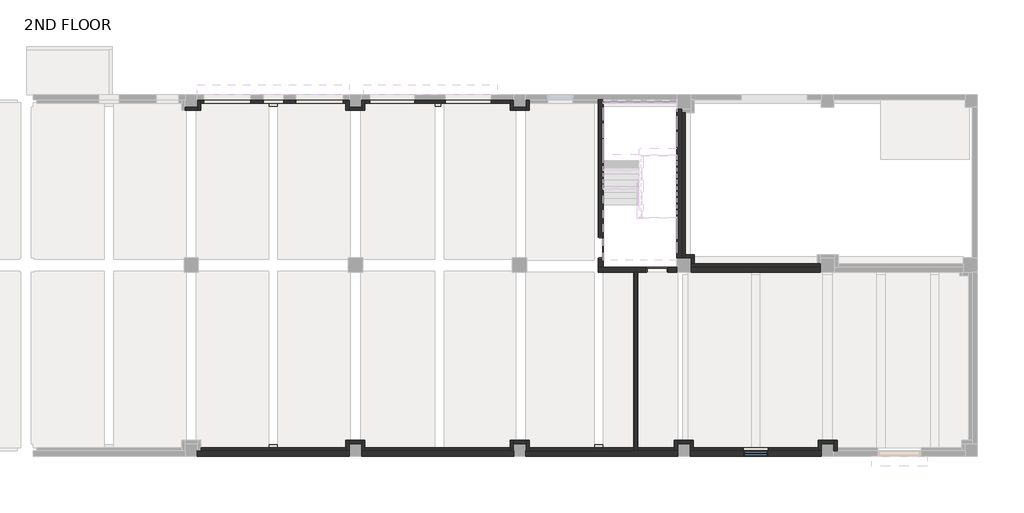
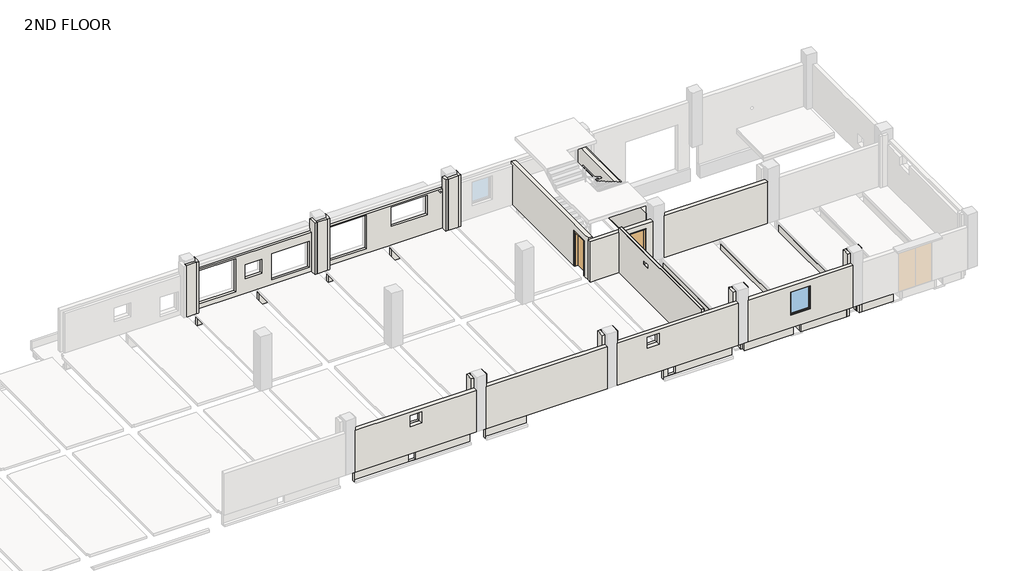
# One storey, part 2 of 7: 60 walls, 2 doors, 1 window.
"""IFC4 building model written with IfcOpenShell, lengths in millimetres."""

import ifcopenshell
import ifcopenshell.guid

model = None  # the IFC model being written
_history = None  # IfcOwnerHistory: only IFC2X3 demands one
_inside = {}  # id of a spatial element -> (the spatial element, [elements in it])
_under = {}  # id of a project, library or spatial element -> (it, [spatial elements below it])
_declared = {}  # id of a project -> (the project, [libraries it declares])
_typed = {}  # id of a type object -> (the type object, [elements of that type])
_made_of = {}  # id of a material, layer set ... -> (it, [elements and type objects made of it])


def new_model(schema):
    """Start an empty IFC model of exactly this schema.

    Asked for "IFC4X3", IfcOpenShell would pick the latest addendum, in which some entities
    have other attributes; the version numbers below select the first issue.
    IFC2X3 requires an IfcOwnerHistory on every rooted entity: one is made here for all.
    """
    global model, _history
    if schema == "IFC4X3":
        model = ifcopenshell.file(schema_version=(4, 3, 0, 0))
    else:
        model = ifcopenshell.file(schema=schema)
    _inside.clear()
    _under.clear()
    _declared.clear()
    _typed.clear()
    _made_of.clear()
    _history = None
    if model.schema == "IFC2X3":
        org = make("IfcOrganization", Name="unknown")
        user = make(
            "IfcPersonAndOrganization",
            ThePerson=make("IfcPerson", FamilyName="unknown"),
            TheOrganization=org,
        )
        app = make(
            "IfcApplication",
            ApplicationDeveloper=org,
            Version="unknown",
            ApplicationFullName="unknown",
            ApplicationIdentifier="unknown",
        )
        _history = make(
            "IfcOwnerHistory",
            OwningUser=user,
            OwningApplication=app,
            ChangeAction="ADDED",
            CreationDate=0,
        )
    return model


def make(cls, **values):
    """One entity of the class cls with the attributes given. An attribute that is None is left unset."""
    return model.create_entity(
        cls, **{name: value for name, value in values.items() if value is not None}
    )


def rooted(cls, **values):
    """An entity with a GlobalId (a new one), such as an element, a storey or a relation."""
    return make(cls, GlobalId=ifcopenshell.guid.new(), OwnerHistory=_history, **values)


def si_unit(unit_type, name, prefix=None):
    """IfcSIUnit, for example si_unit("LENGTHUNIT", "METRE", prefix="MILLI")."""
    return make("IfcSIUnit", UnitType=unit_type, Prefix=prefix, Name=name)


def assignment(units):
    """IfcUnitAssignment: the units of a project."""
    return None if units is None else make("IfcUnitAssignment", Units=units)


def point(xyz):
    """IfcCartesianPoint."""
    return None if xyz is None else make("IfcCartesianPoint", Coordinates=xyz)


def direction(xyz):
    """IfcDirection."""
    return None if xyz is None else make("IfcDirection", DirectionRatios=xyz)


def frame(location, z_axis=None, x_axis=None):
    """IfcAxis2Placement3D, a coordinate frame: its origin and axes. An axis left out is left unset."""
    return make(
        "IfcAxis2Placement3D",
        Location=point(location),
        Axis=direction(z_axis),
        RefDirection=direction(x_axis),
    )


def frame_2d(location, x_axis=None):
    """IfcAxis2Placement2D, a coordinate frame in the plane: its origin and x axis."""
    return make(
        "IfcAxis2Placement2D", Location=point(location), RefDirection=direction(x_axis)
    )


def origin():
    """The frame at (0, 0, 0) with its axes left unset."""
    return frame((0.0, 0.0, 0.0))


def origin_with_axes():
    """The frame at (0, 0, 0) with the z axis (0, 0, 1) and the x axis (1, 0, 0) written out."""
    return frame((0.0, 0.0, 0.0), z_axis=(0.0, 0.0, 1.0), x_axis=(1.0, 0.0, 0.0))


def place(relative_to, where):
    """IfcLocalPlacement: puts the frame where relative to a parent placement (None: the world)."""
    return make(
        "IfcLocalPlacement", PlacementRelTo=relative_to, RelativePlacement=where
    )


def context(
    kind, dimensions, precision=None, world=None, true_north=None, identifier=None
):
    """IfcGeometricRepresentationContext, for example the 3D "Model" context."""
    return make(
        "IfcGeometricRepresentationContext",
        ContextIdentifier=identifier,
        ContextType=kind,
        CoordinateSpaceDimension=dimensions,
        Precision=precision,
        WorldCoordinateSystem=world,
        TrueNorth=true_north,
    )


def project(units=None, contexts=None):
    """IfcProject with its units and contexts."""
    return rooted(
        "IfcProject",
        Name="project",
        RepresentationContexts=contexts,
        UnitsInContext=assignment(units),
    )


def spatial(cls, under=None, at=None, **own):
    """A site, building, storey or space (cls), placed at a placement, below another one or the project."""
    s = rooted(cls, ObjectPlacement=at, **own)
    if under is not None:
        _under.setdefault(under.id(), (under, []))[1].append(s)
    return s


def polyline(points):
    """IfcPolyline through the points."""
    return make("IfcPolyline", Points=[point(p) for p in points])


def circle_curve(where, radius):
    """IfcCircle in the frame where."""
    return make("IfcCircle", Position=where, Radius=radius)


def trimmed(basis, trim1, trim2, sense, master):
    """IfcTrimmedCurve: the piece of a basis curve between two trims."""
    return make(
        "IfcTrimmedCurve",
        BasisCurve=basis,
        Trim1=trim1,
        Trim2=trim2,
        SenseAgreement=sense,
        MasterRepresentation=master,
    )


def segment(curve, same_sense, transition):
    """IfcCompositeCurveSegment."""
    return make(
        "IfcCompositeCurveSegment",
        Transition=transition,
        SameSense=same_sense,
        ParentCurve=curve,
    )


def composite_curve(segments, self_intersect=None):
    """IfcCompositeCurve: segments joined end to end."""
    return make("IfcCompositeCurve", Segments=segments, SelfIntersect=self_intersect)


def outline(outer, holes=None, kind="AREA"):
    """IfcArbitraryClosedProfileDef: a profile drawn as a closed curve; with holes, ...WithVoids."""
    if holes is None:
        return make("IfcArbitraryClosedProfileDef", ProfileType=kind, OuterCurve=outer)
    return make(
        "IfcArbitraryProfileDefWithVoids",
        ProfileType=kind,
        OuterCurve=outer,
        InnerCurves=holes,
    )


def extrude(swept, where, along, depth):
    """IfcExtrudedAreaSolid: the profile swept, set in the frame where, extruded along a direction by depth."""
    return make(
        "IfcExtrudedAreaSolid",
        SweptArea=swept,
        Position=where,
        ExtrudedDirection=direction(along),
        Depth=depth,
    )


def faces_of(points, faces, orient=None, outer=None):
    """IfcFace entities. A face is a list of loops; a loop is a list of indices into points, from 0.

    orient and outer hold one flag for each loop. By default every Orientation is true, the
    first loop of a face is its IfcFaceOuterBound and the others are IfcFaceBound.
    """
    made = []
    for i, loops in enumerate(faces):
        bounds = []
        for j, loop in enumerate(loops):
            is_outer = j == 0 if outer is None else outer[i][j]
            bounds.append(
                make(
                    "IfcFaceOuterBound" if is_outer else "IfcFaceBound",
                    Bound=make("IfcPolyLoop", Polygon=[points[k] for k in loop]),
                    Orientation=True if orient is None else orient[i][j],
                )
            )
        made.append(make("IfcFace", Bounds=bounds))
    return made


def faceted_brep(points, faces, orient=None, outer=None, voids=None):
    """IfcFacetedBrep: a solid bounded by flat faces; with voids (closed shells), ...WithVoids."""
    shared = [point(p) for p in points]
    hull = make("IfcClosedShell", CfsFaces=faces_of(shared, faces, orient, outer))
    if voids is None:
        return make("IfcFacetedBrep", Outer=hull)
    return make(
        "IfcFacetedBrepWithVoids",
        Outer=hull,
        Voids=[
            make(cls, CfsFaces=faces_of(shared, fs, o, b)) for cls, fs, o, b in voids
        ],
    )


def shape(context_of_items, identifier, shape_type, items):
    """IfcShapeRepresentation: the items that make up one representation, for example the "Body"."""
    return make(
        "IfcShapeRepresentation",
        ContextOfItems=context_of_items,
        RepresentationIdentifier=identifier,
        RepresentationType=shape_type,
        Items=items,
    )


def source(mapping_origin, context_of_items, identifier, shape_type, items):
    """IfcRepresentationMap: a shape defined once, which mapped items show again and again."""
    return make(
        "IfcRepresentationMap",
        MappingOrigin=mapping_origin,
        MappedRepresentation=shape(context_of_items, identifier, shape_type, items),
    )


def transform(
    local_origin,
    x_axis=None,
    y_axis=None,
    z_axis=None,
    scale=None,
    scale2=None,
    scale3=None,
    uniform=True,
):
    """IfcCartesianTransformationOperator3D, or its non-uniform kind. x_axis, y_axis, z_axis: its Axis1, 2, 3."""
    if uniform:
        return make(
            "IfcCartesianTransformationOperator3D",
            Axis1=direction(x_axis),
            Axis2=direction(y_axis),
            LocalOrigin=point(local_origin),
            Scale=scale,
            Axis3=direction(z_axis),
        )
    return make(
        "IfcCartesianTransformationOperator3DnonUniform",
        Axis1=direction(x_axis),
        Axis2=direction(y_axis),
        LocalOrigin=point(local_origin),
        Scale=scale,
        Axis3=direction(z_axis),
        Scale2=scale2,
        Scale3=scale3,
    )


def mapped(mapping_source, mapping_target):
    """IfcMappedItem: shows the shape of a source again, moved by a transform."""
    return make(
        "IfcMappedItem", MappingSource=mapping_source, MappingTarget=mapping_target
    )


def made_of(thing, what):
    """Note that an element or type object is made of a material, layer set ...; save() writes the relation."""
    if what is not None:
        _made_of.setdefault(what.id(), (what, []))[1].append(thing)
    return thing


def element(
    cls,
    number,
    at=None,
    inside=None,
    cuts=None,
    type_object=None,
    material=None,
    context=None,
    identifier="Body",
    shape_type=None,
    held_by="IfcProductDefinitionShape",
    body=None,
    shapes=None,
    **own,
):
    """One element of the class cls, such as IfcWall. Its Tag is "e" and its number.

    at: its placement. inside: the storey or other place that contains it. cuts: it is an
    opening in that element (IfcRelVoidsElement). A single representation is given by context,
    identifier, shape_type and body (its items); several are given by shapes. held_by: the class
    of the entity that holds the representations. save() writes the other relations.
    """
    e = rooted(cls, Tag="e%d" % number, ObjectPlacement=at, **own)
    if body is not None:
        shapes = [shape(context, identifier, shape_type, body)]
    if shapes is not None:
        e.Representation = make(held_by, Representations=shapes)
    if inside is not None:
        _inside.setdefault(inside.id(), (inside, []))[1].append(e)
    if cuts is not None:
        rooted(
            "IfcRelVoidsElement", RelatingBuildingElement=cuts, RelatedOpeningElement=e
        )
    if type_object is not None:
        _typed.setdefault(type_object.id(), (type_object, []))[1].append(e)
    return made_of(e, material)


def aggregate(whole, parts):
    """IfcRelAggregates: a whole, such as a stair, and the parts it consists of."""
    return rooted("IfcRelAggregates", RelatingObject=whole, RelatedObjects=parts)


def save(model, path):
    """Write the relations noted so far, then the file.

    IfcRelAggregates (storeys below a building ...), IfcRelContainedInSpatialStructure (elements
    in a storey), IfcRelDefinesByType, IfcRelAssociatesMaterial and IfcRelDeclares: one each for
    every whole, place, type object, material and project.
    """
    for whole, parts in _under.values():
        aggregate(whole, parts)
    for where, things in _inside.values():
        rooted(
            "IfcRelContainedInSpatialStructure",
            RelatedElements=things,
            RelatingStructure=where,
        )
    for kind, things in _typed.values():
        rooted("IfcRelDefinesByType", RelatedObjects=things, RelatingType=kind)
    for what, things in _made_of.values():
        rooted("IfcRelAssociatesMaterial", RelatedObjects=things, RelatingMaterial=what)
    for by, libraries in _declared.values():
        rooted("IfcRelDeclares", RelatingContext=by, RelatedDefinitions=libraries)
    model.write(path)


def single_door_steel_8b0dfbf3(model_context):
    return source(origin(), model_context, "Body", "SolidModel", [
        extrude(outline(polyline([(505.0, -125.0), (-505.0, -125.0), (-505.0, -85.0), (505.0, -85.0), (505.0, -125.0)])), origin_with_axes(), (0.0, 0.0, 1.0), 2235.0),
        faceted_brep([(505.0, -125.0, 0.0), (505.0, -85.0, 0.0), (485.0, -85.0, 0.0), (485.0, 85.0, 0.0), (505.0, 85.0, 0.0), (505.0, 125.0, 0.0), (535.0, 125.0, 0.0), (535.0, -125.0, 0.0), (-505.0, -125.0, 0.0), (-535.0, -125.0, 0.0), (-535.0, 125.0, 0.0), (-505.0, 125.0, 0.0), (-505.0, 85.0, 0.0), (-485.0, 85.0, 0.0), (-485.0, -85.0, 0.0), (-505.0, -85.0, 0.0), (535.0, -125.0, 2265.0), (-535.0, -125.0, 2265.0), (-505.0, -125.0, 2235.0), (505.0, -125.0, 2235.0), (535.0, 125.0, 2265.0), (505.0, 125.0, 2235.0), (-505.0, 125.0, 2235.0), (-535.0, 125.0, 2265.0), (505.0, 85.0, 2235.0), (485.0, 85.0, 2215.0), (-485.0, 85.0, 2215.0), (-505.0, 85.0, 2235.0), (485.0, -85.0, 2215.0), (505.0, -85.0, 2235.0), (-505.0, -85.0, 2235.0), (-485.0, -85.0, 2215.0)], [[[0, 1, 2, 3, 4, 5, 6, 7]], [[8, 9, 10, 11, 12, 13, 14, 15]], [[7, 16, 17, 9, 8, 18, 19, 0]], [[6, 20, 16, 7]], [[5, 21, 22, 11, 10, 23, 20, 6]], [[4, 24, 21, 5]], [[3, 25, 26, 13, 12, 27, 24, 4]], [[2, 28, 25, 3]], [[1, 29, 30, 15, 14, 31, 28, 2]], [[0, 19, 29, 1]], [[18, 8, 15, 30]], [[23, 10, 9, 17]], [[27, 12, 11, 22]], [[31, 14, 13, 26]], [[20, 23, 17, 16]], [[24, 27, 22, 21]], [[28, 31, 26, 25]], [[19, 18, 30, 29]]]),
    ])


def fixed_window_c6e05aa5(model_context):
    return source(origin(), model_context, "Body", "SweptSolid", [
        extrude(outline(polyline([(-550.0, 3.0), (550.0, 3.0), (550.0, -3.0), (-550.0, -3.0), (-550.0, 3.0)])), frame((0.0, 0.0, 850.0), z_axis=(0.0, 0.0, 1.0), x_axis=(1.0, 0.0, 0.0)), (0.0, 0.0, 1.0), 1400.0),
        extrude(outline(polyline([(2300.0, -600.0), (800.0, -600.0), (800.0, 600.0), (2300.0, 600.0), (2300.0, -600.0)]), holes=[polyline([(2250.0, -550.0), (2250.0, 550.0), (850.0, 550.0), (850.0, -550.0), (2250.0, -550.0)])]), frame((0.0, -75.0, 0.0), z_axis=(0.0, 1.0, 0.0), x_axis=(0.0, 0.0, 1.0)), (0.0, 0.0, 1.0), 150.0),
    ])


model = new_model("IFC4")

# Units and contexts
model_context = context("Model", 3, world=origin())
ifc_project = project(units=[si_unit("LENGTHUNIT", "METRE", prefix="MILLI")], contexts=[model_context])

# Site, building, storey
site = spatial("IfcSite", under=ifc_project)
building = spatial("IfcBuilding", under=site)
storey = spatial("IfcBuildingStorey", under=building, Name="2ND FLOOR", Elevation=10600.0)

# Doors
placement = place(None, origin())
single_door_steel_shape = single_door_steel_8b0dfbf3(model_context)
element("IfcDoor", 1, ObjectType="Single Door_Steel : H_DR_AR B12_Door_Single_W1100xH2280_FR 1.0H_FSD-1", at=placement, inside=storey, context=model_context, shape_type="MappedRepresentation", body=[
    mapped(single_door_steel_shape, transform((50950.0, -7150.0, 10600.0), x_axis=(0.0, 1.0, 0.0), y_axis=(-1.0, 0.0, 0.0), z_axis=(0.0, 0.0, 1.0))),
])
element("IfcDoor", 2, ObjectType="Single Door_Steel : H_DR_AR B12_Door_Single_W1100xH2280_FR 1.0H_FSD-1", at=placement, inside=storey, context=model_context, shape_type="MappedRepresentation", body=[
    mapped(single_door_steel_shape, transform((53700.0, -8225.0, 10600.0), x_axis=(-1.0, 0.0, 0.0), y_axis=(0.0, -1.0, 0.0), z_axis=(0.0, 0.0, 1.0))),
])

# Walls
element("IfcWall", 3, ObjectType="H_WA_AR B02_Ext Wall RC-AG_T250_W1", at=placement, inside=storey, context=model_context, shape_type="SweptSolid", body=[
    extrude(outline(polyline([(10600.0, 61700.0), (13300.0, 61700.0), (13300.0, 55300.0), (10600.0, 55300.0), (10600.0, 61700.0)]), holes=[polyline([(11400.0, 59100.0), (11400.0, 57900.0), (12900.0, 57900.0), (12900.0, 59100.0), (11400.0, 59100.0)])]), frame((0.0, -17300.0, 0.0), z_axis=(0.0, 1.0, 0.0), x_axis=(0.0, 0.0, 1.0)), (0.0, 0.0, 1.0), 250.0),
])
element("IfcWall", 4, ObjectType="H_WA_AR B02_Ext Wall RC-AG_T250_W1", at=placement, inside=storey, context=model_context, shape_type="SweptSolid", body=[
    extrude(outline(polyline([(10600.0, 54700.0), (13300.0, 54700.0), (13300.0, 47300.0), (10600.0, 47300.0), (10600.0, 54700.0)]), holes=[polyline([(13070.0, 49860.0), (12350.0, 49860.0), (12350.0, 49140.0), (13070.0, 49140.0), (13070.0, 49860.0)])]), frame((0.0, -17300.0, 0.0), z_axis=(0.0, 1.0, 0.0), x_axis=(0.0, 0.0, 1.0)), (0.0, 0.0, 1.0), 250.0),
])
element("IfcWall", 5, ObjectType="H_WA_AR B02_Ext Wall RC-AG_T250_W1", at=placement, inside=storey, context=model_context, shape_type="SweptSolid", body=[
    extrude(outline(polyline([(39300.0, -17050.0), (46700.0, -17050.0), (46700.0, -17300.0), (39300.0, -17300.0), (39300.0, -17050.0)])), frame((0.0, 0.0, 10600.0), z_axis=(0.0, 0.0, 1.0), x_axis=(1.0, 0.0, 0.0)), (0.0, 0.0, 1.0), 2700.0),
])
element("IfcWall", 6, ObjectType="H_WA_AR B02_Ext Wall RC-AG_T250_W1", at=placement, inside=storey, context=model_context, shape_type="SweptSolid", body=[
    extrude(outline(polyline([(10600.0, 38700.0), (13300.0, 38700.0), (13300.0, 31300.0), (10600.0, 31300.0), (10600.0, 38700.0)]), holes=[polyline([(13070.0, 35360.0), (12350.0, 35360.0), (12350.0, 34640.0), (13070.0, 34640.0), (13070.0, 35360.0)])]), frame((0.0, -17300.0, 0.0), z_axis=(0.0, 1.0, 0.0), x_axis=(0.0, 0.0, 1.0)), (0.0, 0.0, 1.0), 250.0),
])
element("IfcWall", 7, ObjectType="H_WA_AR B02_Int Wall RC-AG_T250_W2", at=placement, inside=storey, context=model_context, shape_type="Brep", body=[
    faceted_brep([(50825.0, -8100.0, 13200.0), (51075.0, -8100.0, 13200.0), (54650.0, -8100.0, 13200.0), (54650.0, -8100.0, 10600.0), (54250.0, -8100.0, 10600.0), (54250.0, -8100.0, 12880.0), (53150.0, -8100.0, 12880.0), (53150.0, -8100.0, 10600.0), (51075.0, -8100.0, 10600.0), (50825.0, -8100.0, 10600.0), (54650.0, -8350.0, 13200.0), (50825.0, -8350.0, 13200.0), (50825.0, -8350.0, 10600.0), (53150.0, -8350.0, 10600.0), (53150.0, -8350.0, 12880.0), (54250.0, -8350.0, 12880.0), (54250.0, -8350.0, 10600.0), (54650.0, -8350.0, 10600.0)], [[[0, 1, 2, 3, 4, 5, 6, 7, 8, 9]], [[10, 11, 12, 13, 14, 15, 16, 17]], [[3, 17, 16, 4]], [[12, 9, 8, 7, 13]], [[2, 1, 0, 11, 10]], [[3, 2, 10, 17]], [[0, 9, 12, 11]], [[6, 14, 13, 7]], [[14, 6, 5, 15]], [[15, 5, 4, 16]]]),
])
element("IfcWall", 8, ObjectType="H_WA_AR B02_Int Wall RC-AG_T250_W2", at=placement, inside=storey, context=model_context, shape_type="Brep", body=[
    faceted_brep([(51075.0, 50.0, 13300.0), (51075.0, -100.0, 13300.0), (51075.0, -7750.0, 13300.0), (51075.0, -8100.0, 13300.0), (51075.0, -8100.0, 13200.0), (51075.0, -8100.0, 10600.0), (51075.0, -7750.0, 10600.0), (51075.0, -7700.0, 10600.0), (51075.0, -7700.0, 12880.0), (51075.0, -6600.0, 12880.0), (51075.0, -6600.0, 10600.0), (51075.0, -100.0, 10600.0), (51075.0, 50.0, 10600.0), (50825.0, -8100.0, 13300.0), (50825.0, -7750.0, 13300.0), (50825.0, 50.0, 13300.0), (50825.0, 50.0, 10600.0), (50825.0, -6600.0, 10600.0), (50825.0, -6600.0, 12880.0), (50825.0, -7700.0, 12880.0), (50825.0, -7700.0, 10600.0), (50825.0, -8100.0, 10600.0), (50825.0, -8100.0, 13200.0)], [[[0, 1, 2, 3, 4, 5, 6, 7, 8, 9, 10, 11, 12]], [[13, 14, 15, 16, 17, 18, 19, 20, 21, 22]], [[5, 21, 20, 7, 6]], [[16, 12, 11, 10, 17]], [[3, 2, 1, 0, 15, 14, 13]], [[5, 4, 3, 13, 22, 21]], [[0, 12, 16, 15]], [[9, 18, 17, 10]], [[18, 9, 8, 19]], [[19, 8, 7, 20]]]),
])
element("IfcWall", 9, ObjectType="H_WA_AR B02_Int Wall RC-AG_T250_W2", at=placement, inside=storey, context=model_context, shape_type="SweptSolid", body=[
    extrude(outline(polyline([(54650.0, -7650.0), (54650.0, -400.0), (54900.0, -400.0), (54900.0, -7650.0), (54650.0, -7650.0)])), frame((0.0, 0.0, 10600.0), z_axis=(0.0, 0.0, 1.0), x_axis=(1.0, 0.0, 0.0)), (0.0, 0.0, 1.0), 2700.0),
])
element("IfcWall", 10, ObjectType="H_WA_AR B02_Int Wall RC-AG_T250_W2", at=placement, inside=storey, context=model_context, shape_type="SweptSolid", body=[
    extrude(outline(polyline([(61650.0, -8350.0), (55350.0, -8350.0), (55350.0, -8100.0), (61650.0, -8100.0), (61650.0, -8350.0)])), frame((0.0, 0.0, 10600.0), z_axis=(0.0, 0.0, 1.0), x_axis=(1.0, 0.0, 0.0)), (0.0, 0.0, 1.0), 2700.0),
])
element("IfcWall", 11, ObjectType="H_WA_AR B02_Ext Wall DY-IN_T154", at=placement, inside=storey, context=model_context, shape_type="SweptSolid", body=[
    extrude(outline(polyline([(10600.0, 31464.0), (10600.0, 38536.0), (13136.0, 38536.0), (13136.0, 31464.0), (10600.0, 31464.0)]), holes=[polyline([(13070.0, 35360.0), (12350.0, 35360.0), (12350.0, 34640.0), (13070.0, 34640.0), (13070.0, 35360.0)])]), frame((0.0, -17040.0, 0.0), z_axis=(0.0, 1.0, 0.0), x_axis=(0.0, 0.0, 1.0)), (0.0, 0.0, 1.0), 154.0),
])
element("IfcWall", 12, ObjectType="H_WA_AR B02_Ext Wall DY-IN_T154", at=placement, inside=storey, context=model_context, shape_type="Brep", body=[
    faceted_brep([(38690.0, -17040.0, 10600.0), (38690.0, -16690.0, 10600.0), (38690.0, -16536.0, 10600.0), (38690.0, -16536.0, 13920.0), (38690.0, -16690.0, 13920.0), (38690.0, -17040.0, 13920.0), (38536.0, -17040.0, 10600.0), (38536.0, -17040.0, 13155.0), (38536.0, -17040.0, 13920.0), (38536.0, -16890.0, 13920.0), (38536.0, -16736.0, 13920.0), (38536.0, -16536.0, 13920.0), (38536.0, -16536.0, 10600.0), (38536.0, -16886.0, 10600.0)], [[[0, 1, 2, 3, 4, 5]], [[6, 7, 8, 9, 10, 11, 12, 13]], [[2, 1, 0, 6, 13, 12]], [[5, 4, 3, 11, 10, 9, 8]], [[3, 2, 12, 11]], [[0, 5, 8, 7, 6]]]),
])
element("IfcWall", 13, ObjectType="H_WA_AR B02_Ext Wall DY-IN_T154", at=placement, inside=storey, context=model_context, shape_type="SweptSolid", body=[
    extrude(outline(polyline([(39310.0, -16690.0), (38690.0, -16690.0), (38690.0, -16536.0), (39310.0, -16536.0), (39310.0, -16690.0)])), frame((0.0, 0.0, 10600.0), z_axis=(0.0, 0.0, 1.0), x_axis=(1.0, 0.0, 0.0)), (0.0, 0.0, 1.0), 3320.0),
])
element("IfcWall", 14, ObjectType="H_WA_AR B02_Ext Wall DY-IN_T154", at=placement, inside=storey, context=model_context, shape_type="Brep", body=[
    faceted_brep([(39310.0, -16536.0, 10600.0), (39310.0, -16690.0, 10600.0), (39310.0, -17040.0, 10600.0), (39310.0, -17040.0, 13920.0), (39310.0, -16690.0, 13920.0), (39310.0, -16536.0, 13920.0), (39464.0, -16536.0, 10600.0), (39464.0, -16536.0, 13920.0), (39464.0, -16736.0, 13920.0), (39464.0, -16890.0, 13920.0), (39464.0, -17040.0, 13920.0), (39464.0, -17040.0, 13136.0), (39464.0, -17040.0, 10600.0), (39464.0, -16886.0, 10600.0)], [[[0, 1, 2, 3, 4, 5]], [[6, 7, 8, 9, 10, 11, 12, 13]], [[2, 1, 0, 6, 13, 12]], [[5, 4, 3, 10, 9, 8, 7]], [[0, 5, 7, 6]], [[3, 2, 12, 11, 10]]]),
])
element("IfcWall", 15, ObjectType="H_WA_AR B02_Ext Wall DY-IN_T154", at=placement, inside=storey, context=model_context, shape_type="SweptSolid", body=[
    extrude(outline(polyline([(46536.0, -17040.0), (39464.0, -17040.0), (39464.0, -16886.0), (46536.0, -16886.0), (46536.0, -17040.0)])), frame((0.0, 0.0, 10600.0), z_axis=(0.0, 0.0, 1.0), x_axis=(1.0, 0.0, 0.0)), (0.0, 0.0, 1.0), 2536.0),
])
element("IfcWall", 16, ObjectType="H_WA_AR B02_Ext Wall DY-IN_T154", at=placement, inside=storey, context=model_context, shape_type="Brep", body=[
    faceted_brep([(46690.0, -17040.0, 10600.0), (46690.0, -16690.0, 10600.0), (46690.0, -16536.0, 10600.0), (46690.0, -16536.0, 13920.0), (46690.0, -16690.0, 13920.0), (46690.0, -17040.0, 13920.0), (46536.0, -17040.0, 10600.0), (46536.0, -17040.0, 13155.0), (46536.0, -17040.0, 13920.0), (46536.0, -16536.0, 13920.0), (46536.0, -16536.0, 10600.0), (46536.0, -16886.0, 10600.0)], [[[0, 1, 2, 3, 4, 5]], [[6, 7, 8, 9, 10, 11]], [[2, 1, 0, 6, 11, 10]], [[5, 4, 3, 9, 8]], [[3, 2, 10, 9]], [[0, 5, 8, 7, 6]]]),
])
element("IfcWall", 17, ObjectType="H_WA_AR B02_Ext Wall DY-IN_T154", at=placement, inside=storey, context=model_context, shape_type="SweptSolid", body=[
    extrude(outline(polyline([(47310.0, -16690.0), (46690.0, -16690.0), (46690.0, -16536.0), (47310.0, -16536.0), (47310.0, -16690.0)])), frame((0.0, 0.0, 10600.0), z_axis=(0.0, 0.0, 1.0), x_axis=(1.0, 0.0, 0.0)), (0.0, 0.0, 1.0), 3320.0),
])
element("IfcWall", 18, ObjectType="H_WA_AR B02_Ext Wall DY-IN_T154", at=placement, inside=storey, context=model_context, shape_type="Brep", body=[
    faceted_brep([(47310.0, -16536.0, 10600.0), (47310.0, -16690.0, 10600.0), (47310.0, -17040.0, 10600.0), (47310.0, -17040.0, 13920.0), (47310.0, -16690.0, 13920.0), (47310.0, -16536.0, 13920.0), (47464.0, -16536.0, 10600.0), (47464.0, -16536.0, 13920.0), (47464.0, -17040.0, 13920.0), (47464.0, -17040.0, 13155.0), (47464.0, -17040.0, 10600.0), (47464.0, -16886.0, 10600.0)], [[[0, 1, 2, 3, 4, 5]], [[6, 7, 8, 9, 10, 11]], [[2, 1, 0, 6, 11, 10]], [[5, 4, 3, 8, 7]], [[0, 5, 7, 6]], [[3, 2, 10, 9, 8]]]),
])
element("IfcWall", 19, ObjectType="H_WA_AR B02_Ext Wall DY-IN_T154", at=placement, inside=storey, context=model_context, shape_type="SweptSolid", body=[
    extrude(outline(polyline([(10600.0, 47464.0), (10600.0, 52557.0), (13136.0, 52557.0), (13136.0, 47464.0), (10600.0, 47464.0)]), holes=[polyline([(13070.0, 49860.0), (12350.0, 49860.0), (12350.0, 49140.0), (13070.0, 49140.0), (13070.0, 49860.0)])]), frame((0.0, -17040.0, 0.0), z_axis=(0.0, 1.0, 0.0), x_axis=(0.0, 0.0, 1.0)), (0.0, 0.0, 1.0), 154.0),
])
element("IfcWall", 20, ObjectType="H_WA_AR B02_Ext Wall DY-IN_T154", at=placement, inside=storey, context=model_context, shape_type="Brep", body=[
    faceted_brep([(54690.0, -17040.0, 10600.0), (54690.0, -16690.0, 10600.0), (54690.0, -16536.0, 10600.0), (54690.0, -16536.0, 13920.0), (54690.0, -16690.0, 13920.0), (54690.0, -17040.0, 13920.0), (54536.0, -17040.0, 10600.0), (54536.0, -17040.0, 13155.0), (54536.0, -17040.0, 13920.0), (54536.0, -16890.0, 13920.0), (54536.0, -16736.0, 13920.0), (54536.0, -16536.0, 13920.0), (54536.0, -16536.0, 10600.0), (54536.0, -16886.0, 10600.0)], [[[0, 1, 2, 3, 4, 5]], [[6, 7, 8, 9, 10, 11, 12, 13]], [[2, 1, 0, 6, 13, 12]], [[5, 4, 3, 11, 10, 9, 8]], [[3, 2, 12, 11]], [[0, 5, 8, 7, 6]]]),
])
element("IfcWall", 21, ObjectType="H_WA_AR B02_Ext Wall DY-IN_T154", at=placement, inside=storey, context=model_context, shape_type="SweptSolid", body=[
    extrude(outline(polyline([(55310.0, -16690.0), (54690.0, -16690.0), (54690.0, -16536.0), (55310.0, -16536.0), (55310.0, -16690.0)])), frame((0.0, 0.0, 10600.0), z_axis=(0.0, 0.0, 1.0), x_axis=(1.0, 0.0, 0.0)), (0.0, 0.0, 1.0), 3320.0),
])
element("IfcWall", 22, ObjectType="H_WA_AR B02_Ext Wall DY-IN_T154", at=placement, inside=storey, context=model_context, shape_type="Brep", body=[
    faceted_brep([(55310.0, -16536.0, 10600.0), (55310.0, -16690.0, 10600.0), (55310.0, -17040.0, 10600.0), (55310.0, -17040.0, 13920.0), (55310.0, -16690.0, 13920.0), (55310.0, -16536.0, 13920.0), (55464.0, -16536.0, 10600.0), (55464.0, -16536.0, 13920.0), (55464.0, -16736.0, 13920.0), (55464.0, -16890.0, 13920.0), (55464.0, -17040.0, 13920.0), (55464.0, -17040.0, 13155.0), (55464.0, -17040.0, 10600.0), (55464.0, -16886.0, 10600.0)], [[[0, 1, 2, 3, 4, 5]], [[6, 7, 8, 9, 10, 11, 12, 13]], [[2, 1, 0, 6, 13, 12]], [[5, 4, 3, 10, 9, 8, 7]], [[0, 5, 7, 6]], [[3, 2, 12, 11, 10]]]),
])
element("IfcWall", 23, ObjectType="H_WA_AR B02_Ext Wall DY-IN_T154", at=placement, inside=storey, context=model_context, shape_type="SweptSolid", body=[
    extrude(outline(polyline([(10600.0, 55464.0), (10600.0, 61536.0), (13136.0, 61536.0), (13136.0, 55464.0), (10600.0, 55464.0)]), holes=[polyline([(12900.0, 59100.0), (11400.0, 59100.0), (11400.0, 57900.0), (12900.0, 57900.0), (12900.0, 59100.0)])]), frame((0.0, -17040.0, 0.0), z_axis=(0.0, 1.0, 0.0), x_axis=(0.0, 0.0, 1.0)), (0.0, 0.0, 1.0), 154.0),
])
element("IfcWall", 24, ObjectType="H_WA_AR B02_Int Wall MA_T150", at=placement, inside=storey, context=model_context, shape_type="SweptSolid", body=[
    extrude(outline(polyline([(-17050.0, 10600.0), (-17050.0, 13500.0), (-8350.0, 13500.0), (-8350.0, 10600.0), (-17050.0, 10600.0)]), holes=[polyline([(-11000.0, 12950.0), (-11400.0, 12950.0), (-11400.0, 12750.0), (-11000.0, 12750.0), (-11000.0, 12950.0)])]), frame((52575.0, 0.0, 0.0), z_axis=(1.0, 0.0, 0.0), x_axis=(0.0, 1.0, 0.0)), (0.0, 0.0, 1.0), 150.0),
])
element("IfcWall", 25, ObjectType="H_WA_AR B02_Ext Wall DY-IN_T154", at=placement, inside=storey, context=model_context, shape_type="SweptSolid", body=[
    extrude(outline(polyline([(54536.0, -17040.0), (52743.0, -17040.0), (52743.0, -16886.0), (54536.0, -16886.0), (54536.0, -17040.0)])), frame((0.0, 0.0, 10600.0), z_axis=(0.0, 0.0, 1.0), x_axis=(1.0, 0.0, 0.0)), (0.0, 0.0, 1.0), 2536.0),
])
element("IfcWall", 26, ObjectType="H_WA_AR B02_Ext Wall DY-IN_T154", at=placement, inside=storey, context=model_context, shape_type="Brep", body=[
    faceted_brep([(61690.0, -17040.0, 10600.0), (61690.0, -16690.0, 10600.0), (61690.0, -16536.0, 10600.0), (61690.0, -16536.0, 13920.0), (61690.0, -16690.0, 13920.0), (61690.0, -17040.0, 13920.0), (61536.0, -17040.0, 10600.0), (61536.0, -17040.0, 13155.0), (61536.0, -17040.0, 13920.0), (61536.0, -16890.0, 13920.0), (61536.0, -16736.0, 13920.0), (61536.0, -16536.0, 13920.0), (61536.0, -16536.0, 10600.0), (61536.0, -16886.0, 10600.0)], [[[0, 1, 2, 3, 4, 5]], [[6, 7, 8, 9, 10, 11, 12, 13]], [[2, 1, 0, 6, 13, 12]], [[5, 4, 3, 11, 10, 9, 8]], [[3, 2, 12, 11]], [[0, 5, 8, 7, 6]]]),
])
element("IfcWall", 27, ObjectType="H_WA_AR B02_Ext Wall DY-IN_T154", at=placement, inside=storey, context=model_context, shape_type="SweptSolid", body=[
    extrude(outline(polyline([(62310.0, -16690.0), (61690.0, -16690.0), (61690.0, -16536.0), (62310.0, -16536.0), (62310.0, -16690.0)])), frame((0.0, 0.0, 10600.0), z_axis=(0.0, 0.0, 1.0), x_axis=(1.0, 0.0, 0.0)), (0.0, 0.0, 1.0), 3320.0),
])
element("IfcWall", 28, ObjectType="H_WA_AR B02_Ext Wall DY-IN_T154", at=placement, inside=storey, context=model_context, shape_type="Brep", body=[
    faceted_brep([(62310.0, -16536.0, 10600.0), (62310.0, -16690.0, 10600.0), (62310.0, -17040.0, 10600.0), (62310.0, -17040.0, 13155.0), (62310.0, -16890.0, 13155.0), (62310.0, -16890.0, 13920.0), (62310.0, -16690.0, 13920.0), (62310.0, -16536.0, 13920.0), (62464.0, -16536.0, 10600.0), (62464.0, -16536.0, 13920.0), (62464.0, -16736.0, 13920.0), (62464.0, -16890.0, 13920.0), (62464.0, -16890.0, 13155.0), (62464.0, -17040.0, 13155.0), (62464.0, -17040.0, 13136.0), (62464.0, -17040.0, 10600.0), (62464.0, -16886.0, 10600.0)], [[[0, 1, 2, 3, 4, 5, 6, 7]], [[8, 9, 10, 11, 12, 13, 14, 15, 16]], [[2, 1, 0, 8, 16, 15]], [[7, 6, 5, 11, 10, 9]], [[0, 7, 9, 8]], [[12, 4, 3, 13]], [[3, 2, 15, 14, 13]], [[5, 4, 12, 11]]]),
])
element("IfcWall", 29, ObjectType="H_WA_AR B02_Ext Wall DY-IN_T154", at=placement, inside=storey, context=model_context, shape_type="SweptSolid", body=[
    extrude(outline(polyline([(31310.0, -464.0), (30690.0, -464.0), (30690.0, -310.0), (31310.0, -310.0), (31310.0, -464.0)])), frame((0.0, 0.0, 10600.0), z_axis=(0.0, 0.0, 1.0), x_axis=(1.0, 0.0, 0.0)), (0.0, 0.0, 1.0), 3320.0),
])
element("IfcWall", 30, ObjectType="H_WA_AR B02_Ext Wall DY-IN_T154", at=placement, inside=storey, context=model_context, shape_type="Brep", body=[
    faceted_brep([(31464.0, -464.0, 10600.0), (31464.0, -114.0, 10600.0), (31464.0, 40.0, 10600.0), (31464.0, 40.0, 13136.0), (31464.0, 40.0, 13920.0), (31464.0, -110.0, 13920.0), (31464.0, -264.0, 13920.0), (31464.0, -464.0, 13920.0), (31310.0, -464.0, 10600.0), (31310.0, -464.0, 13920.0), (31310.0, -310.0, 13920.0), (31310.0, 40.0, 13920.0), (31310.0, 40.0, 10600.0), (31310.0, -310.0, 10600.0)], [[[0, 1, 2, 3, 4, 5, 6, 7]], [[8, 9, 10, 11, 12, 13]], [[2, 1, 0, 8, 13, 12]], [[7, 6, 5, 4, 11, 10, 9]], [[0, 7, 9, 8]], [[4, 3, 2, 12, 11]]]),
])
element("IfcWall", 31, ObjectType="H_WA_AR B02_Ext Wall DY-IN_T154", at=placement, inside=storey, context=model_context, shape_type="SweptSolid", body=[
    extrude(outline(polyline([(10600.0, 31464.0), (10600.0, 38536.0), (13136.0, 38536.0), (13136.0, 31464.0), (10600.0, 31464.0)]), holes=[polyline([(10900.0, 36100.0), (12600.0, 36100.0), (12600.0, 38400.0), (10900.0, 38400.0), (10900.0, 36100.0)]), polyline([(10900.0, 31600.0), (13050.0, 31600.0), (13050.0, 33900.0), (10900.0, 33900.0), (10900.0, 31600.0)]), polyline([(11550.0, 34500.0), (12450.0, 34500.0), (12450.0, 35500.0), (11550.0, 35500.0), (11550.0, 34500.0)])]), frame((0.0, -114.0, 0.0), z_axis=(0.0, 1.0, 0.0), x_axis=(0.0, 0.0, 1.0)), (0.0, 0.0, 1.0), 154.0),
])
element("IfcWall", 32, ObjectType="H_WA_AR B02_Ext Wall DY-IN_T154", at=placement, inside=storey, context=model_context, shape_type="Brep", body=[
    faceted_brep([(38536.0, 40.0, 10600.0), (38536.0, -114.0, 10600.0), (38536.0, -464.0, 10600.0), (38536.0, -464.0, 13920.0), (38536.0, -264.0, 13920.0), (38536.0, -110.0, 13920.0), (38536.0, 40.0, 13920.0), (38536.0, 40.0, 13136.0), (38690.0, 40.0, 10600.0), (38690.0, 40.0, 13920.0), (38690.0, -310.0, 13920.0), (38690.0, -464.0, 13920.0), (38690.0, -464.0, 10600.0), (38690.0, -310.0, 10600.0)], [[[0, 1, 2, 3, 4, 5, 6, 7]], [[8, 9, 10, 11, 12, 13]], [[2, 1, 0, 8, 13, 12]], [[6, 5, 4, 3, 11, 10, 9]], [[3, 2, 12, 11]], [[0, 7, 6, 9, 8]]]),
])
element("IfcWall", 33, ObjectType="H_WA_AR B02_Ext Wall DY-IN_T154", at=placement, inside=storey, context=model_context, shape_type="SweptSolid", body=[
    extrude(outline(polyline([(39310.0, -464.0), (38690.0, -464.0), (38690.0, -310.0), (39310.0, -310.0), (39310.0, -464.0)])), frame((0.0, 0.0, 10600.0), z_axis=(0.0, 0.0, 1.0), x_axis=(1.0, 0.0, 0.0)), (0.0, 0.0, 1.0), 3320.0),
])
element("IfcWall", 34, ObjectType="H_WA_AR B02_Ext Wall DY-IN_T154", at=placement, inside=storey, context=model_context, shape_type="Brep", body=[
    faceted_brep([(39464.0, -464.0, 10600.0), (39464.0, -114.0, 10600.0), (39464.0, 40.0, 10600.0), (39464.0, 40.0, 13136.0), (39464.0, 40.0, 13920.0), (39464.0, -110.0, 13920.0), (39464.0, -264.0, 13920.0), (39464.0, -464.0, 13920.0), (39310.0, -464.0, 10600.0), (39310.0, -464.0, 13920.0), (39310.0, -310.0, 13920.0), (39310.0, 40.0, 13920.0), (39310.0, 40.0, 10600.0), (39310.0, -310.0, 10600.0)], [[[0, 1, 2, 3, 4, 5, 6, 7]], [[8, 9, 10, 11, 12, 13]], [[2, 1, 0, 8, 13, 12]], [[7, 6, 5, 4, 11, 10, 9]], [[0, 7, 9, 8]], [[4, 3, 2, 12, 11]]]),
])
element("IfcWall", 35, ObjectType="H_WA_AR B02_Ext Wall DY-IN_T154", at=placement, inside=storey, context=model_context, shape_type="SweptSolid", body=[
    extrude(outline(polyline([(10600.0, 39464.0), (10600.0, 46536.0), (13136.0, 46536.0), (13136.0, 39464.0), (10600.0, 39464.0)]), holes=[composite_curve([segment(trimmed(circle_curve(frame_2d((12955.0, 46436.0)), 25.0), [point((12955.0, 46461.0))], [point((12955.0, 46411.0))], True, "CARTESIAN"), True, "CONTINUOUS"), segment(trimmed(circle_curve(frame_2d((12955.0, 46436.0)), 25.0), [point((12955.0, 46411.0))], [point((12955.0, 46461.0))], True, "CARTESIAN"), True, "CONTINUOUS")], self_intersect=False), polyline([(11800.0, 43400.0), (13050.0, 43400.0), (13050.0, 45600.0), (11800.0, 45600.0), (11800.0, 43400.0)]), polyline([(10900.0, 39700.0195059), (13050.0, 39700.0195059), (13050.0, 41900.0195059), (10900.0, 41900.0195059), (10900.0, 39700.0195059)])]), frame((0.0, -114.0, 0.0), z_axis=(0.0, 1.0, 0.0), x_axis=(0.0, 0.0, 1.0)), (0.0, 0.0, 1.0), 154.0),
])
element("IfcWall", 36, ObjectType="H_WA_AR B02_Ext Wall DY-IN_T154", at=placement, inside=storey, context=model_context, shape_type="Brep", body=[
    faceted_brep([(46536.0, 40.0, 10600.0), (46536.0, -114.0, 10600.0), (46536.0, -464.0, 10600.0), (46536.0, -464.0, 13920.0), (46536.0, -264.0, 13920.0), (46536.0, -110.0, 13920.0), (46536.0, -110.0, 13155.0), (46536.0, 40.0, 13155.0), (46536.0, 40.0, 13136.0), (46690.0, 40.0, 10600.0), (46690.0, 40.0, 13155.0), (46690.0, -110.0, 13155.0), (46690.0, -110.0, 13920.0), (46690.0, -310.0, 13920.0), (46690.0, -464.0, 13920.0), (46690.0, -464.0, 10600.0), (46690.0, -310.0, 10600.0)], [[[0, 1, 2, 3, 4, 5, 6, 7, 8]], [[9, 10, 11, 12, 13, 14, 15, 16]], [[2, 1, 0, 9, 16, 15]], [[5, 4, 3, 14, 13, 12]], [[3, 2, 15, 14]], [[6, 11, 10, 7]], [[0, 8, 7, 10, 9]], [[6, 5, 12, 11]]]),
])
element("IfcWall", 37, ObjectType="H_WA_AR B02_Ext Wall DY-IN_T154", at=placement, inside=storey, context=model_context, shape_type="SweptSolid", body=[
    extrude(outline(polyline([(47310.0, -464.0), (46690.0, -464.0), (46690.0, -310.0), (47310.0, -310.0), (47310.0, -464.0)])), frame((0.0, 0.0, 10600.0), z_axis=(0.0, 0.0, 1.0), x_axis=(1.0, 0.0, 0.0)), (0.0, 0.0, 1.0), 3320.0),
])
element("IfcWall", 38, ObjectType="H_WA_AR B02_Ext Wall DY-IN_T154", at=placement, inside=storey, context=model_context, shape_type="Brep", body=[
    faceted_brep([(47464.0, -464.0, 10600.0), (47464.0, -114.0, 10600.0), (47464.0, 40.0, 10600.0), (47464.0, 40.0, 13136.0), (47464.0, 40.0, 13920.0), (47464.0, -110.0, 13920.0), (47464.0, -264.0, 13920.0), (47464.0, -464.0, 13920.0), (47310.0, -464.0, 10600.0), (47310.0, -464.0, 13920.0), (47310.0, -310.0, 13920.0), (47310.0, 40.0, 13920.0), (47310.0, 40.0, 10600.0), (47310.0, -310.0, 10600.0)], [[[0, 1, 2, 3, 4, 5, 6, 7]], [[8, 9, 10, 11, 12, 13]], [[2, 1, 0, 8, 13, 12]], [[7, 6, 5, 4, 11, 10, 9]], [[0, 7, 9, 8]], [[4, 3, 2, 12, 11]]]),
])
element("IfcWall", 39, ObjectType="H_WA_AR B02_Ext Wall DY-IN_T154", at=placement, inside=storey, context=model_context, shape_type="SweptSolid", body=[
    extrude(outline(polyline([(-7640.0, 10735.0), (-7640.0, 13155.0), (-7486.0, 13155.0), (-7486.0, 13136.0), (-564.0, 13136.0), (-564.0, 10754.0), (-7486.0, 10754.0), (-7486.0, 10735.0), (-7640.0, 10735.0)])), frame((54910.0, 0.0, 0.0), z_axis=(1.0, 0.0, 0.0), x_axis=(0.0, 1.0, 0.0)), (0.0, 0.0, 1.0), 154.0),
])
element("IfcWall", 40, ObjectType="H_WA_AR B02_Ext Wall DY-IN_T154", at=placement, inside=storey, context=model_context, shape_type="Brep", body=[
    faceted_brep([(55064.0, -7640.0, 10600.0), (55360.0, -7640.0, 10600.0), (55514.0, -7640.0, 10600.0), (55514.0, -7640.0, 13766.0), (55360.0, -7640.0, 13766.0), (55064.0, -7640.0, 13766.0), (55064.0, -7640.0, 13155.0), (55064.0, -7640.0, 10735.0), (55064.0, -7486.0, 10600.0), (55064.0, -7486.0, 10735.0), (55064.0, -7486.0, 10754.0), (55064.0, -7486.0, 13136.0), (55064.0, -7486.0, 13155.0), (55064.0, -7486.0, 13766.0), (55514.0, -7486.0, 13766.0), (55514.0, -7486.0, 10600.0)], [[[0, 1, 2, 3, 4, 5, 6, 7]], [[8, 9, 10, 11, 12, 13, 14, 15]], [[2, 1, 0, 8, 15]], [[5, 4, 3, 14, 13]], [[0, 7, 6, 5, 13, 12, 11, 10, 9, 8]], [[2, 15, 14, 3]]]),
])
element("IfcWall", 41, ObjectType="H_WA_AR B02_Ext Wall DY-IN_T154", at=placement, inside=storey, context=model_context, shape_type="Brep", body=[
    faceted_brep([(55360.0, -7640.0, 13766.0), (55360.0, -7640.0, 10600.0), (55360.0, -7936.0, 10600.0), (55360.0, -7936.0, 10735.0), (55360.0, -7936.0, 13155.0), (55360.0, -7936.0, 13766.0), (55514.0, -7640.0, 10600.0), (55514.0, -7640.0, 13766.0), (55514.0, -7936.0, 13766.0), (55514.0, -7936.0, 13155.0), (55514.0, -7936.0, 13136.0), (55514.0, -7936.0, 10754.0), (55514.0, -7936.0, 10735.0), (55514.0, -7936.0, 10600.0)], [[[0, 1, 2, 3, 4, 5]], [[6, 7, 8, 9, 10, 11, 12, 13]], [[2, 1, 6, 13]], [[0, 5, 8, 7]], [[5, 4, 3, 2, 13, 12, 11, 10, 9, 8]], [[0, 7, 6, 1]]]),
])
element("IfcWall", 42, ObjectType="H_WA_AR B02_Ext Wall DY-IN_T154", at=placement, inside=storey, context=model_context, shape_type="SweptSolid", body=[
    extrude(outline(polyline([(13155.0, 55360.0), (10735.0, 55360.0), (10735.0, 55514.0), (10754.0, 55514.0), (10754.0, 61486.0), (10735.0, 61486.0), (10735.0, 61640.0), (13155.0, 61640.0), (13155.0, 61486.0), (13136.0, 61486.0), (13136.0, 55514.0), (13155.0, 55514.0), (13155.0, 55360.0)])), frame((0.0, -8090.0, 0.0), z_axis=(0.0, 1.0, 0.0), x_axis=(0.0, 0.0, 1.0)), (0.0, 0.0, 1.0), 154.0),
])
element("IfcWall", 43, ObjectType="H_WA_AR B02_Ext Wall DY-IN_T154", at=placement, inside=storey, context=model_context, shape_type="Brep", body=[
    faceted_brep([(55160.0, -564.0, 10735.0), (55160.0, -564.0, 10600.0), (55160.0, -564.0, 9800.0), (55160.0, -564.0, 9665.0), (55160.0, -7486.0, 9665.0), (55160.0, -7486.0, 9800.0), (55160.0, -7486.0, 10600.0), (55160.0, -7486.0, 10735.0), (55314.0, -564.0, 9665.0), (55314.0, -564.0, 10735.0), (55314.0, -7486.0, 10735.0), (55314.0, -7486.0, 9665.0)], [[[0, 1, 2, 3, 4, 5, 6, 7]], [[8, 9, 10, 11]], [[4, 3, 8, 11]], [[0, 7, 10, 9]], [[0, 9, 8, 3, 2, 1]], [[4, 11, 10, 7, 6, 5]]]),
])
element("IfcWall", 44, ObjectType="H_WA_AR_B07_Int Wall_Plaster_T18", at=placement, inside=storey, context=model_context, shape_type="SweptSolid", body=[
    extrude(outline(polyline([(-8350.0, 10600.0), (-17050.0, 10600.0), (-17050.0, 13500.0), (-8350.0, 13500.0), (-8350.0, 10600.0)]), holes=[polyline([(-11000.0, 12950.0), (-11400.0, 12950.0), (-11400.0, 12750.0), (-11000.0, 12750.0), (-11000.0, 12950.0)])]), frame((52557.0, 0.0, 0.0), z_axis=(1.0, 0.0, 0.0), x_axis=(0.0, 1.0, 0.0)), (0.0, 0.0, 1.0), 18.0),
])
element("IfcWall", 45, ObjectType="H_WA_AR_B07_Int Wall_Plaster_T18", at=placement, inside=storey, context=model_context, shape_type="SweptSolid", body=[
    extrude(outline(polyline([(-17050.0, 10600.0), (-17050.0, 13500.0), (-8350.0, 13500.0), (-8350.0, 10600.0), (-17050.0, 10600.0)]), holes=[polyline([(-11000.0, 12950.0), (-11400.0, 12950.0), (-11400.0, 12750.0), (-11000.0, 12750.0), (-11000.0, 12950.0)])]), frame((52725.0, 0.0, 0.0), z_axis=(1.0, 0.0, 0.0), x_axis=(0.0, 1.0, 0.0)), (0.0, 0.0, 1.0), 18.0),
])
element("IfcWall", 46, ObjectType="H_CE_AR_B09_Souns Absorbing_100T_C7", at=placement, inside=storey, context=model_context, shape_type="Brep", body=[
    faceted_brep([(55300.0, -16700.0, 9800.0), (55300.0, -16536.0, 9800.0), (55300.0, -8469.0, 9800.0), (55300.0, -8469.0, 10350.0), (55300.0, -16536.0, 10350.0), (55300.0, -16700.0, 10350.0), (55200.0, -16700.0, 9800.0), (55200.0, -16700.0, 10350.0), (55200.0, -8469.0, 10350.0), (55200.0, -8469.0, 9800.0)], [[[0, 1, 2, 3, 4, 5]], [[6, 7, 8, 9]], [[2, 1, 0, 6, 9]], [[5, 4, 3, 8, 7]], [[0, 5, 7, 6]], [[3, 2, 9, 8]]]),
])
element("IfcWall", 47, ObjectType="H_CE_AR_B09_Souns Absorbing_100T_C7", at=placement, inside=storey, context=model_context, shape_type="Brep", body=[
    faceted_brep([(55300.0, -16900.0, 9800.0), (58275.0, -16900.0, 9800.0), (58275.0, -16900.0, 10350.0), (55300.0, -16900.0, 10350.0), (55300.0, -16800.0, 9800.0), (55300.0, -16800.0, 10350.0), (55464.0, -16800.0, 10350.0), (58175.0, -16800.0, 10350.0), (58275.0, -16800.0, 10350.0), (58275.0, -16800.0, 9800.0), (58175.0, -16800.0, 9800.0), (55464.0, -16800.0, 9800.0)], [[[0, 1, 2, 3]], [[4, 5, 6, 7, 8, 9, 10, 11]], [[1, 0, 4, 11, 10, 9]], [[3, 2, 8, 7, 6, 5]], [[0, 3, 5, 4]], [[2, 1, 9, 8]]]),
])
element("IfcWall", 48, ObjectType="H_CE_AR_B09_Souns Absorbing_100T_C7 2", at=placement, inside=storey, context=model_context, shape_type="Brep", body=[
    faceted_brep([(55464.0, -16800.0, 9800.0), (55464.0, -16536.0, 9800.0), (55464.0, -16536.0, 10350.0), (55464.0, -16800.0, 10350.0), (55300.0, -16800.0, 9800.0), (55300.0, -16800.0, 10350.0), (55300.0, -16700.0, 10350.0), (55300.0, -16536.0, 10350.0), (55300.0, -16536.0, 9800.0), (55300.0, -16700.0, 9800.0)], [[[0, 1, 2, 3]], [[4, 5, 6, 7, 8, 9]], [[1, 0, 4, 9, 8]], [[2, 1, 8, 7]], [[3, 2, 7, 6, 5]], [[0, 3, 5, 4]]]),
])
element("IfcWall", 49, ObjectType="H_CE_AR_B09_Souns Absorbing_100T_C7", at=placement, inside=storey, context=model_context, shape_type="SweptSolid", body=[
    extrude(outline(polyline([(58825.0, -8469.0), (58825.0, -16800.0), (58725.0, -16800.0), (58725.0, -8469.0), (58825.0, -8469.0)])), frame((0.0, 0.0, 9800.0), z_axis=(0.0, 0.0, 1.0), x_axis=(1.0, 0.0, 0.0)), (0.0, 0.0, 1.0), 550.0),
])
element("IfcWall", 50, ObjectType="H_CE_AR_B09_Souns Absorbing_100T_C7", at=placement, inside=storey, context=model_context, shape_type="SweptSolid", body=[
    extrude(outline(polyline([(58275.0, -8469.0), (58275.0, -16800.0), (58175.0, -16800.0), (58175.0, -8469.0), (58275.0, -8469.0)])), frame((0.0, 0.0, 9800.0), z_axis=(0.0, 0.0, 1.0), x_axis=(1.0, 0.0, 0.0)), (0.0, 0.0, 1.0), 550.0),
])
element("IfcWall", 51, ObjectType="H_CE_AR_B09_Souns Absorbing_100T_C7", at=placement, inside=storey, context=model_context, shape_type="Brep", body=[
    faceted_brep([(58725.0, -16900.0, 9800.0), (61536.0, -16900.0, 9800.0), (61536.0, -16900.0, 10350.0), (58725.0, -16900.0, 10350.0), (58725.0, -16800.0, 9800.0), (58725.0, -16800.0, 10350.0), (58825.0, -16800.0, 10350.0), (61536.0, -16800.0, 10350.0), (61536.0, -16800.0, 9800.0), (58825.0, -16800.0, 9800.0)], [[[0, 1, 2, 3]], [[4, 5, 6, 7, 8, 9]], [[1, 0, 4, 9, 8]], [[3, 2, 7, 6, 5]], [[2, 1, 8, 7]], [[0, 3, 5, 4]]]),
])
element("IfcWall", 52, ObjectType="H_CE_AR_B09_Souns Absorbing_100T_C7 2", at=placement, inside=storey, context=model_context, shape_type="Brep", body=[
    faceted_brep([(62464.0, -16900.0, 9800.0), (62464.0, -16800.0, 9800.0), (62464.0, -16536.0, 9800.0), (62464.0, -16536.0, 10350.0), (62464.0, -16800.0, 10350.0), (62464.0, -16900.0, 10350.0), (62300.0, -16900.0, 9800.0), (62300.0, -16900.0, 10350.0), (62300.0, -16700.0, 10350.0), (62300.0, -16700.0, 9800.0), (62350.0, -16700.0, 9800.0), (62350.0, -16536.0, 9800.0), (62350.0, -16536.0, 10350.0), (62350.0, -16700.0, 10350.0)], [[[0, 1, 2, 3, 4, 5]], [[6, 7, 8, 9]], [[2, 1, 0, 6, 9, 10, 11]], [[3, 2, 11, 12]], [[5, 4, 3, 12, 13, 8, 7]], [[0, 5, 7, 6]], [[10, 13, 12, 11]], [[13, 10, 9, 8]]]),
])
element("IfcWall", 53, ObjectType="H_CE_AR_B09_Souns Absorbing_100T_C7 2", at=placement, inside=storey, context=model_context, shape_type="Brep", body=[
    faceted_brep([(61700.0, -16900.0, 10350.0), (61700.0, -16900.0, 9800.0), (61700.0, -16700.0, 9800.0), (61700.0, -16700.0, 10350.0), (61536.0, -16536.0, 9800.0), (61536.0, -16800.0, 9800.0), (61536.0, -16900.0, 9800.0), (61536.0, -16900.0, 10350.0), (61536.0, -16800.0, 10350.0), (61536.0, -16536.0, 10350.0), (61650.0, -16536.0, 9800.0), (61650.0, -16700.0, 9800.0), (61650.0, -16536.0, 10350.0), (61650.0, -16700.0, 10350.0)], [[[0, 1, 2, 3]], [[4, 5, 6, 7, 8, 9]], [[6, 5, 4, 10, 11, 2, 1]], [[4, 9, 12, 10]], [[9, 8, 7, 0, 3, 13, 12]], [[1, 0, 7, 6]], [[13, 11, 10, 12]], [[11, 13, 3, 2]]]),
])
element("IfcWall", 54, ObjectType="H_CE_AR_B09_Souns Absorbing_100T_C7", at=placement, inside=storey, context=model_context, shape_type="Brep", body=[
    faceted_brep([(64375.0, -16800.0, 9800.0), (64275.0, -16800.0, 9800.0), (62464.0, -16800.0, 9800.0), (62464.0, -16800.0, 10350.0), (64275.0, -16800.0, 10350.0), (64375.0, -16800.0, 10350.0), (64375.0, -16900.0, 9800.0), (64375.0, -16900.0, 10350.0), (62464.0, -16900.0, 10350.0), (62464.0, -16900.0, 9800.0)], [[[0, 1, 2, 3, 4, 5]], [[6, 7, 8, 9]], [[2, 1, 0, 6, 9]], [[5, 4, 3, 8, 7]], [[3, 2, 9, 8]], [[0, 5, 7, 6]]]),
])
element("IfcWall", 55, ObjectType="H_CE_AR_B09_Souns Absorbing_100T_C7", at=placement, inside=storey, context=model_context, shape_type="Brep", body=[
    faceted_brep([(61750.0, -16700.0, 9800.0), (61750.0, -8469.0, 9800.0), (61750.0, -8469.0, 10350.0), (61750.0, -16700.0, 10350.0), (61650.0, -16700.0, 9800.0), (61650.0, -16700.0, 10350.0), (61650.0, -16536.0, 10350.0), (61650.0, -8469.0, 10350.0), (61650.0, -8469.0, 9800.0), (61650.0, -16536.0, 9800.0), (61700.0, -16700.0, 9800.0), (61700.0, -16700.0, 10350.0)], [[[0, 1, 2, 3]], [[4, 5, 6, 7, 8, 9]], [[1, 0, 10, 4, 9, 8]], [[3, 2, 7, 6, 5, 11]], [[0, 3, 11, 5, 4, 10]], [[2, 1, 8, 7]]]),
])
element("IfcWall", 56, ObjectType="H_CE_AR_B09_Souns Absorbing_100T_C7", at=placement, inside=storey, context=model_context, shape_type="Brep", body=[
    faceted_brep([(62350.0, -16700.0, 9800.0), (62350.0, -16536.0, 9800.0), (62350.0, -8469.0, 9800.0), (62350.0, -8469.0, 10350.0), (62350.0, -16536.0, 10350.0), (62350.0, -16700.0, 10350.0), (62250.0, -16700.0, 9800.0), (62250.0, -16700.0, 10350.0), (62250.0, -8469.0, 10350.0), (62250.0, -8469.0, 9800.0), (62300.0, -16700.0, 9800.0), (62300.0, -16700.0, 10350.0)], [[[0, 1, 2, 3, 4, 5]], [[6, 7, 8, 9]], [[2, 1, 0, 10, 6, 9]], [[5, 4, 3, 8, 7, 11]], [[0, 5, 11, 7, 6, 10]], [[3, 2, 9, 8]]]),
])
element("IfcWall", 57, ObjectType="H_WA_AR B02_Ext Wall DY-IN_T154", at=placement, inside=storey, context=model_context, shape_type="Brep", body=[
    faceted_brep([(31464.0, -16890.0, 9655.0), (38536.0, -16890.0, 9655.0), (38536.0, -16890.0, 9790.0), (38536.0, -16890.0, 10450.0), (35225.0, -16890.0, 10450.0), (35225.0, -16890.0, 9800.0), (34775.0, -16890.0, 9800.0), (34775.0, -16890.0, 10450.0), (31464.0, -16890.0, 10450.0), (31464.0, -16890.0, 9790.0), (38536.0, -16736.0, 9655.0), (31464.0, -16736.0, 9655.0), (31464.0, -16736.0, 10450.0), (34775.0, -16736.0, 10450.0), (34775.0, -16736.0, 9800.0), (35225.0, -16736.0, 9800.0), (35225.0, -16736.0, 10450.0), (38536.0, -16736.0, 10450.0), (31464.0, -16886.0, 9655.0), (38536.0, -16886.0, 9655.0)], [[[0, 1, 2, 3, 4, 5, 6, 7, 8, 9]], [[10, 11, 12, 13, 14, 15, 16, 17]], [[1, 0, 18, 11, 10, 19]], [[12, 8, 7, 13]], [[3, 17, 16, 4]], [[0, 9, 8, 12, 11, 18]], [[3, 2, 1, 19, 10, 17]], [[6, 14, 13, 7]], [[14, 6, 5, 15]], [[15, 5, 4, 16]]]),
])
element("IfcWall", 58, ObjectType="H_WA_AR B02_Ext Wall DY-IN_T154", at=placement, inside=storey, context=model_context, shape_type="Brep", body=[
    faceted_brep([(39464.0, -16890.0, 9655.0), (41975.0, -16890.0, 9655.0), (41975.0, -16890.0, 9790.0), (41975.0, -16890.0, 10450.0), (39464.0, -16890.0, 10450.0), (39464.0, -16890.0, 9790.0), (39464.0, -16736.0, 9655.0), (39464.0, -16736.0, 10450.0), (41975.0, -16736.0, 10450.0), (41975.0, -16736.0, 9655.0)], [[[0, 1, 2, 3, 4, 5]], [[6, 7, 8, 9]], [[1, 0, 6, 9]], [[3, 2, 1, 9, 8]], [[4, 3, 8, 7]], [[0, 5, 4, 7, 6]]]),
])
element("IfcWall", 59, ObjectType="H_WA_AR B02_Ext Wall DY-IN_T154", at=placement, inside=storey, context=model_context, shape_type="Brep", body=[
    faceted_brep([(50343.0, -16890.0, 9655.0), (54536.0, -16890.0, 9655.0), (54536.0, -16890.0, 9790.0), (54536.0, -16890.0, 10450.0), (51075.0, -16890.0, 10450.0), (51075.0, -16890.0, 9800.0), (50625.0, -16890.0, 9800.0), (50625.0, -16890.0, 10450.0), (50343.0, -16890.0, 10450.0), (50343.0, -16890.0, 9790.0), (54536.0, -16736.0, 9655.0), (50343.0, -16736.0, 9655.0), (50343.0, -16736.0, 10450.0), (50625.0, -16736.0, 10450.0), (50625.0, -16736.0, 9800.0), (51075.0, -16736.0, 9800.0), (51075.0, -16736.0, 10450.0), (54536.0, -16736.0, 10450.0)], [[[0, 1, 2, 3, 4, 5, 6, 7, 8, 9]], [[10, 11, 12, 13, 14, 15, 16, 17]], [[1, 0, 11, 10]], [[3, 2, 1, 10, 17]], [[3, 17, 16, 4]], [[12, 8, 7, 13]], [[0, 9, 8, 12, 11]], [[6, 14, 13, 7]], [[14, 6, 5, 15]], [[15, 5, 4, 16]]]),
])
element("IfcWall", 60, ObjectType="H_WA_AR B02_Ext Wall DY-IN_T154", at=placement, inside=storey, context=model_context, shape_type="Brep", body=[
    faceted_brep([(31464.0, -264.0, 9655.0), (38536.0, -264.0, 9655.0), (38536.0, -264.0, 10450.0), (35225.0, -264.0, 10450.0), (35225.0, -264.0, 9800.0), (34775.0, -264.0, 9800.0), (34775.0, -264.0, 10450.0), (31464.0, -264.0, 10450.0), (38536.0, -110.0, 9655.0), (31464.0, -110.0, 9655.0), (31464.0, -110.0, 9790.0), (31464.0, -110.0, 10450.0), (34775.0, -110.0, 10450.0), (34775.0, -110.0, 9800.0), (35225.0, -110.0, 9800.0), (35225.0, -110.0, 10450.0), (38536.0, -110.0, 10450.0), (38536.0, -110.0, 9790.0)], [[[0, 1, 2, 3, 4, 5, 6, 7]], [[8, 9, 10, 11, 12, 13, 14, 15, 16, 17]], [[1, 0, 9, 8]], [[11, 7, 6, 12]], [[2, 16, 15, 3]], [[0, 7, 11, 10, 9]], [[2, 1, 8, 17, 16]], [[5, 13, 12, 6]], [[13, 5, 4, 14]], [[14, 4, 3, 15]]]),
])
element("IfcWall", 61, ObjectType="H_WA_AR B02_Ext Wall DY-IN_T154", at=placement, inside=storey, context=model_context, shape_type="Brep", body=[
    faceted_brep([(39464.0, -264.0, 9655.0), (43157.0, -264.0, 9655.0), (43157.0, -264.0, 9800.0), (42875.0, -264.0, 9800.0), (42875.0, -264.0, 10450.0), (39464.0, -264.0, 10450.0), (43157.0, -110.0, 9655.0), (39464.0, -110.0, 9655.0), (39464.0, -110.0, 9790.0), (39464.0, -110.0, 10450.0), (42875.0, -110.0, 10450.0), (42875.0, -110.0, 9800.0), (43157.0, -110.0, 9800.0), (43157.0, -110.0, 9790.0)], [[[0, 1, 2, 3, 4, 5]], [[6, 7, 8, 9, 10, 11, 12, 13]], [[1, 0, 7, 6]], [[9, 5, 4, 10]], [[0, 5, 9, 8, 7]], [[1, 6, 13, 12, 2]], [[11, 3, 2, 12]], [[3, 11, 10, 4]]]),
])
element("IfcWall", 62, ObjectType="H_WA_AR B02_Ext Wall DY-IN_T154", at=placement, inside=storey, context=model_context, shape_type="Brep", body=[
    faceted_brep([(43325.0, -264.0, 9655.0), (46536.0, -264.0, 9655.0), (46536.0, -264.0, 10450.0), (43325.0, -264.0, 10450.0), (43325.0, -110.0, 9655.0), (43325.0, -110.0, 9790.0), (43325.0, -110.0, 10450.0), (46536.0, -110.0, 10450.0), (46536.0, -110.0, 9790.0), (46536.0, -110.0, 9655.0)], [[[0, 1, 2, 3]], [[4, 5, 6, 7, 8, 9]], [[1, 0, 4, 9]], [[3, 2, 7, 6]], [[2, 1, 9, 8, 7]], [[0, 3, 6, 5, 4]]]),
])

# Window
fixed_window_shape = fixed_window_c6e05aa5(model_context)
element("IfcWindow", 63, ObjectType="Fixed Window : H_WD_AR_B11_Fix_Steel Window_SG_W1200xH1500_AW-2", at=placement, inside=storey, context=model_context, shape_type="MappedRepresentation", body=[
    mapped(fixed_window_shape, transform((58500.0, -17175.0, 10600.0), x_axis=(-1.0, 0.0, 0.0), y_axis=(0.0, -1.0, 0.0), z_axis=(0.0, 0.0, 1.0))),
])

save(model, "model.ifc")

# Revit data of these elements
# Type "Single Door_Steel : H_DR_AR B12_Door_Single_W1100xH2280_FR 1.0H_FSD-1"
#   Type Mark = "441"
#   Analytic Construction = "<None>"
#   프레임 투영 외부. = 25 mm
#   프레임 투영 내부. = 25 mm
#   프레임 폭 = 75 mm
#   Height = 2280 mm
#   Width = 1100 mm
